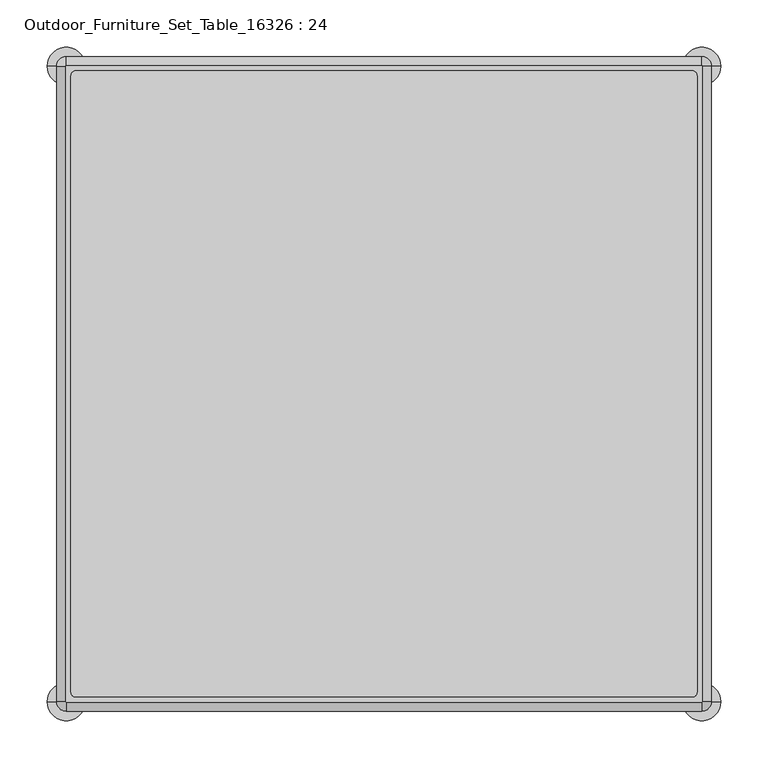
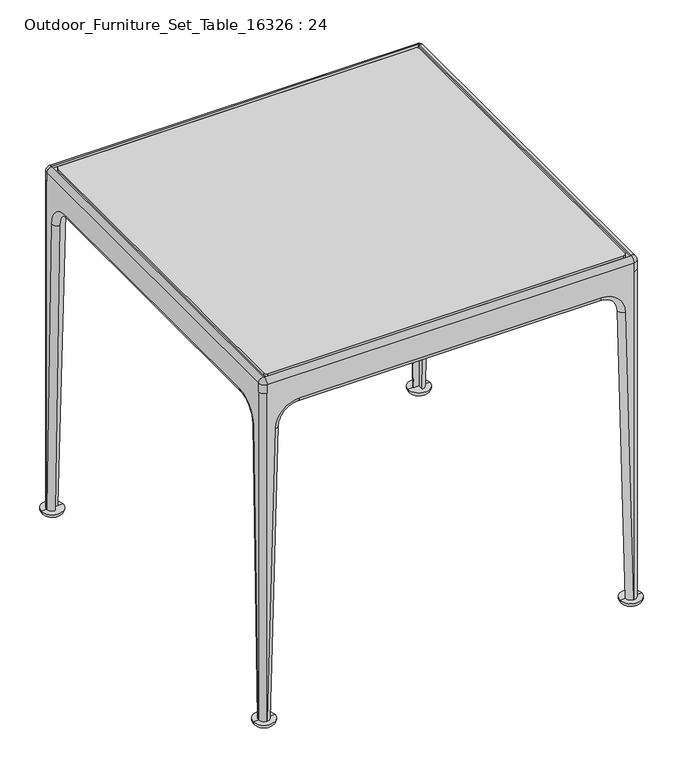
"""IFC4 building model written with IfcOpenShell, lengths in millimetres: furniture geometry, Outdoor_Furniture_Set_Table_16326 : 24."""

from ifc_helpers import new_model, si_unit, point, frame, frame_2d, origin, place, context, project, spatial, polyline, circle_curve, ellipse_curve, trimmed, segment, composite_curve, outline, extrude, source, transform, mapped, element, save
from ifc_brep_helpers import plane_surface, cylinder_surface, revolved_surface, advanced_brep


def outdoor_furniture_set_table_16326_24_87b8b4b7(model_context):
    return source(origin(), model_context, "Body", "SolidModel", [
        extrude(outline(polyline([(337.0, 337.0), (337.0, -337.0), (-337.0, -337.0), (-337.0, 337.0), (337.0, 337.0)])), frame((0.0, 0.0, 645.0), z_axis=(0.0, 0.0, 1.0), x_axis=(1.0, 0.0, 0.0)), (0.0, 0.0, 1.0), 20.0),
        advanced_brep(
        [(-336.0, 346.0, 10.0), (-326.0034268, 336.0, 9.7382305), (-336.0, 336.0, 10.0), (-321.3050379, 346.0, 571.1779627), (-311.3084646, 336.0, 570.9161932), (-276.3204583, 336.0, 605.0), (276.3204583, 336.0, 605.0), (311.3084646, 336.0, 570.9161932), (326.0034268, 336.0, 9.7382305), (336.0, 336.0, 10.0), (336.0, 336.0, 645.0), (-336.0, 336.0, 645.0), (-276.3204583, 346.0, 615.0), (276.3204583, 346.0, 615.0), (321.3050379, 346.0, 571.1779627), (336.0, 346.0, 10.0), (-336.0, 346.0, 645.0), (-336.0, 346.0, 661.0), (336.0, 346.0, 661.0), (336.0, 346.0, 645.0), (-337.0, -336.0, 645.0), (-336.0, -337.0, 645.0), (336.0, -337.0, 645.0), (337.0, -336.0, 645.0), (337.0, 336.0, 645.0), (336.0, 337.0, 645.0), (-336.0, 337.0, 645.0), (-337.0, 336.0, 645.0), (336.0, -336.0, 645.0), (-336.0, -336.0, 645.0), (-336.0, -346.0, 661.0), (-346.0, -336.0, 661.0), (-346.0, -336.0, 645.0), (-336.0, -346.0, 645.0), (-336.0, -337.0, 670.0), (-337.0, -336.0, 670.0), (-336.0, -346.0, 10.0), (-321.3050273, -346.0, 571.1783664), (-276.3204583, -346.0, 615.0), (276.3204583, -346.0, 615.0), (321.3050273, -346.0, 571.1783664), (336.0, -346.0, 10.0), (336.0, -346.0, 645.0), (336.0, -346.0, 661.0), (336.0, -337.0, 670.0), (346.0, -336.0, 645.0), (346.0, -336.0, 661.0), (337.0, -336.0, 670.0), (346.0, -336.0, 10.0), (346.0, -321.3050379, 571.1779627), (346.0, -276.3204583, 615.0), (346.0, 276.3204583, 615.0), (346.0, 321.3050379, 571.1779627), (346.0, 336.0, 10.0), (346.0, 336.0, 645.0), (346.0, 336.0, 661.0), (337.0, 336.0, 670.0), (336.0, 337.0, 670.0), (-336.0, 337.0, 670.0), (-346.0, 336.0, 645.0), (-346.0, 336.0, 661.0), (-337.0, 336.0, 670.0), (-346.0, 336.0, 10.0), (-346.0, 321.3050273, 571.1783665), (-346.0, 276.3208622, 615.0), (-346.0, -276.3208622, 615.0), (-346.0, -321.3050273, 571.1783665), (-346.0, -336.0, 10.0), (-336.0, -326.0034268, 9.7382305), (-336.0, -336.0, 10.0), (-336.0, -311.3084541, 570.916597), (-336.0, -276.3208622, 605.0), (-336.0, 276.3208622, 605.0), (-336.0, 311.3084541, 570.916597), (-336.0, 326.0034268, 9.7382305), (326.0034268, -336.0, 9.7382305), (336.0, -336.0, 10.0), (311.3084564, -336.0, 570.9165072), (276.3204583, -336.0, 605.0), (-276.3204583, -336.0, 605.0), (-311.3084564, -336.0, 570.9165072), (-326.0034268, -336.0, 9.7382305), (336.0, 326.0034268, 9.7382305), (336.0, 311.3084646, 570.9161932), (336.0, 276.3204583, 605.0), (336.0, -276.3204583, 605.0), (336.0, -311.3084646, 570.9161932), (336.0, -326.0034268, 9.7382305)],
        [
            (0, 1, circle_curve(frame((-336.0, 336.0, 10.0), z_axis=(-0.026176948307801547, 0.0, -0.9996573249755591), x_axis=(0.9996573249755591, 0.0, -0.026176948307801547)), 10.0)),
            (1, 2),
            (2, 0),
            (0, 3),
            (3, 4, circle_curve(frame((-321.3050379, 336.0, 571.1779627), z_axis=(-0.026176948307801547, 0.0, -0.9996573249755591), x_axis=(0.9996573249755591, 0.0, -0.026176948307801547)), 10.0)),
            (4, 1),
            (4, 5, circle_curve(frame((-276.3204583, 336.0, 570.0), z_axis=(0.0, 1.0, 0.0), x_axis=(-0.9996573249743329, 0.0, 0.026176948354628502)), 35.0)),
            (5, 6),
            (6, 7, circle_curve(frame((276.3204583, 336.0, 570.0), z_axis=(0.0, 1.0, 0.0), x_axis=(0.0, 0.0, 1.0)), 35.0)),
            (7, 8),
            (8, 9),
            (9, 10),
            (10, 11),
            (11, 2),
            (3, 12, circle_curve(frame((-276.3204583, 346.0, 570.0), z_axis=(0.0, 1.0, 0.0), x_axis=(-0.9996573249743329, 0.0, 0.026176948354628502)), 45.0)),
            (12, 5, circle_curve(frame((-276.3204583, 336.0, 615.0), z_axis=(-1.0, 0.0, 0.0), x_axis=(0.0, 0.0, -1.0)), 10.0)),
            (12, 13),
            (13, 6, circle_curve(frame((276.3204583, 336.0, 615.0), z_axis=(-1.0, 0.0, 0.0), x_axis=(0.0, 0.0, -1.0)), 10.0)),
            (13, 14, circle_curve(frame((276.3204583, 346.0, 570.0), z_axis=(0.0, 1.0, 0.0), x_axis=(0.0, 0.0, 1.0)), 45.0)),
            (14, 7, circle_curve(frame((321.3050379, 336.0, 571.1779627), z_axis=(-0.02617694835452745, 0.0, 0.9996573249743356), x_axis=(-0.9996573249743356, 0.0, -0.02617694835452745)), 10.0)),
            (8, 15, circle_curve(frame((336.0, 336.0, 10.0), z_axis=(0.026176948307803226, 0.0, -0.9996573249755591), x_axis=(-0.9996573249755591, 0.0, -0.026176948307803226)), 10.0)),
            (15, 9),
            (14, 15),
            (0, 16),
            (16, 17),
            (17, 18),
            (18, 19),
            (19, 15),
            (20, 21, circle_curve(frame((-336.0, -336.0, 645.0), z_axis=(0.0, 0.0, 1.0), x_axis=(-1.0, 0.0, 0.0)), 1.0)),
            (21, 22),
            (22, 23, circle_curve(frame((336.0, -336.0, 645.0), z_axis=(0.0, 0.0, 1.0), x_axis=(0.0, -1.0, 0.0)), 1.0)),
            (23, 24),
            (24, 25, circle_curve(frame((336.0, 336.0, 645.0), z_axis=(0.0, 0.0, 1.0), x_axis=(1.0, 0.0, 0.0)), 1.0)),
            (25, 26),
            (26, 27, circle_curve(frame((-336.0, 336.0, 645.0), z_axis=(0.0, 0.0, 1.0), x_axis=(0.0, 1.0, 0.0)), 1.0)),
            (27, 20),
            (10, 28),
            (28, 29),
            (29, 11),
            (30, 31, circle_curve(frame((-336.0, -336.0, 661.0), z_axis=(0.0, 0.0, -1.0), x_axis=(-1.0, 0.0, 0.0)), 10.0)),
            (31, 32),
            (32, 33, circle_curve(frame((-336.0, -336.0, 645.0), z_axis=(0.0, 0.0, 1.0), x_axis=(-1.0, 0.0, 0.0)), 10.0)),
            (33, 30),
            (30, 34, circle_curve(frame((-336.0, -337.0, 661.0), z_axis=(-1.0, 0.0, 0.0), x_axis=(0.0, 1.0, 0.0)), 9.0)),
            (34, 35, circle_curve(frame((-336.0, -336.0, 670.0), z_axis=(0.0, 0.0, -1.0), x_axis=(-1.0, 0.0, 0.0)), 1.0)),
            (35, 31, circle_curve(frame((-337.0, -336.0, 661.0), z_axis=(0.0, -1.0, 0.0), x_axis=(1.0, 0.0, 0.0)), 9.0)),
            (33, 36),
            (36, 37),
            (37, 38, circle_curve(frame((-276.3204583, -346.0, 570.0), z_axis=(0.0, 1.0, 0.0), x_axis=(0.0, 0.0, 1.0)), 45.0)),
            (38, 39),
            (39, 40, circle_curve(frame((276.3204583, -346.0, 570.0), z_axis=(0.0, 1.0, 0.0), x_axis=(0.9996570900025821, 0.0, 0.026185920025262065)), 45.0)),
            (40, 41),
            (41, 42),
            (42, 43),
            (43, 30),
            (43, 44, circle_curve(frame((336.0, -337.0, 661.0), z_axis=(-1.0, 0.0, 0.0), x_axis=(0.0, 1.0, 0.0)), 9.0)),
            (44, 34),
            (42, 45, circle_curve(frame((336.0, -336.0, 645.0), z_axis=(0.0, 0.0, 1.0), x_axis=(0.0, -1.0, 0.0)), 10.0)),
            (45, 46),
            (46, 43, circle_curve(frame((336.0, -336.0, 661.0), z_axis=(0.0, 0.0, -1.0), x_axis=(0.0, -1.0, 0.0)), 10.0)),
            (46, 47, circle_curve(frame((337.0, -336.0, 661.0), z_axis=(0.0, -1.0, 0.0), x_axis=(-1.0, 0.0, 0.0)), 9.0)),
            (47, 44, circle_curve(frame((336.0, -336.0, 670.0), z_axis=(0.0, 0.0, -1.0), x_axis=(0.0, -1.0, 0.0)), 1.0)),
            (45, 48),
            (48, 49),
            (49, 50, circle_curve(frame((346.0, -276.3204583, 570.0), z_axis=(-1.0, 0.0, 0.0), x_axis=(0.0, 0.0, 1.0)), 45.0)),
            (50, 51),
            (51, 52, circle_curve(frame((346.0, 276.3204583, 570.0), z_axis=(-1.0, 0.0, 0.0), x_axis=(0.0, 0.9996573249744088, 0.026176948351728707)), 45.0)),
            (52, 53),
            (53, 54),
            (54, 55),
            (55, 46),
            (55, 56, circle_curve(frame((337.0, 336.0, 661.0), z_axis=(0.0, -1.0, 0.0), x_axis=(-1.0, 0.0, 0.0)), 9.0)),
            (56, 47),
            (54, 19, circle_curve(frame((336.0, 336.0, 645.0), z_axis=(0.0, 0.0, 1.0), x_axis=(1.0, 0.0, 0.0)), 10.0)),
            (18, 55, circle_curve(frame((336.0, 336.0, 661.0), z_axis=(0.0, 0.0, -1.0), x_axis=(1.0, 0.0, 0.0)), 10.0)),
            (18, 57, circle_curve(frame((336.0, 337.0, 661.0), z_axis=(1.0, 0.0, 0.0), x_axis=(0.0, -1.0, 0.0)), 9.0)),
            (57, 56, circle_curve(frame((336.0, 336.0, 670.0), z_axis=(0.0, 0.0, -1.0), x_axis=(1.0, 0.0, 0.0)), 1.0)),
            (17, 58, circle_curve(frame((-336.0, 337.0, 661.0), z_axis=(1.0, 0.0, 0.0), x_axis=(0.0, -1.0, 0.0)), 9.0)),
            (58, 57),
            (16, 59, circle_curve(frame((-336.0, 336.0, 645.0), z_axis=(0.0, 0.0, 1.0), x_axis=(0.0, 1.0, 0.0)), 10.0)),
            (59, 60),
            (60, 17, circle_curve(frame((-336.0, 336.0, 661.0), z_axis=(0.0, 0.0, -1.0), x_axis=(0.0, 1.0, 0.0)), 10.0)),
            (60, 61, circle_curve(frame((-337.0, 336.0, 661.0), z_axis=(0.0, 1.0, 0.0), x_axis=(1.0, 0.0, 0.0)), 9.0)),
            (61, 58, circle_curve(frame((-336.0, 336.0, 670.0), z_axis=(0.0, 0.0, -1.0), x_axis=(0.0, 1.0, 0.0)), 1.0)),
            (31, 60),
            (59, 62),
            (62, 63),
            (63, 64, circle_curve(frame((-346.0, 276.3208622, 570.0004146), z_axis=(1.0, 0.0, 0.0), x_axis=(0.0, 0.0, 1.0)), 44.9995854)),
            (64, 65),
            (65, 66, circle_curve(frame((-346.0, -276.3208622, 570.0004146), z_axis=(1.0, 0.0, 0.0), x_axis=(0.0, -0.9996573249744442, 0.026176948350383943)), 44.9995854)),
            (66, 67),
            (67, 32),
            (35, 61),
            (34, 21),
            (20, 35),
            (44, 22),
            (47, 23),
            (56, 24),
            (57, 25),
            (58, 26),
            (61, 27),
            (67, 68, circle_curve(frame((-336.0, -336.0, 10.0), z_axis=(0.0, -0.0261769483078763, -0.9996573249755573), x_axis=(0.0, -0.9996573249755573, 0.0261769483078763)), 10.0)),
            (68, 69),
            (69, 67),
            (66, 70, circle_curve(frame((-336.0, -321.3050273, 571.1783665), z_axis=(0.0, -0.0261769483078763, -0.9996573249755573), x_axis=(0.0, -0.9996573249755573, 0.0261769483078763)), 10.0)),
            (70, 68),
            (70, 71, circle_curve(frame((-336.0, -276.3208622, 570.0004146), z_axis=(-1.0, 0.0, 0.0), x_axis=(0.0, -0.9996573249744442, 0.026176948350383943)), 34.9995854)),
            (71, 72),
            (72, 73, circle_curve(frame((-336.0, 276.3208622, 570.0004146), z_axis=(-1.0, 0.0, 0.0), x_axis=(0.0, 0.0, 1.0)), 34.9995854)),
            (73, 74),
            (74, 2),
            (29, 69),
            (65, 71, circle_curve(frame((-336.0, -276.3208622, 615.0), z_axis=(0.0, -1.0, 0.0), x_axis=(0.0, 0.0, 1.0)), 10.0)),
            (64, 72, circle_curve(frame((-336.0, 276.3208622, 615.0), z_axis=(0.0, -1.0, 0.0), x_axis=(0.0, 0.0, 1.0)), 10.0)),
            (63, 73, circle_curve(frame((-336.0, 321.3050273, 571.1783665), z_axis=(0.0, -0.026176948350192727, 0.9996573249744491), x_axis=(0.0, 0.9996573249744491, 0.026176948350192727)), 10.0)),
            (74, 62, circle_curve(frame((-336.0, 336.0, 10.0), z_axis=(0.0, 0.026176948307874842, -0.9996573249755573), x_axis=(0.0, 0.9996573249755573, 0.026176948307874842)), 10.0)),
            (62, 2),
            (41, 75, circle_curve(frame((336.0, -336.0, 10.0), z_axis=(0.02617694831120199, 0.0, -0.9996573249754701), x_axis=(-0.9996573249754701, 0.0, -0.02617694831120199)), 10.0)),
            (75, 76),
            (76, 41),
            (40, 77, circle_curve(frame((321.3050273, -336.0, 571.1783664), z_axis=(0.026185920025262068, 0.0, -0.9996570900025821), x_axis=(-0.9996570900025821, 0.0, -0.026185920025262068)), 10.0)),
            (77, 75),
            (77, 78, circle_curve(frame((276.3204583, -336.0, 570.0), z_axis=(0.0, -1.0, 0.0), x_axis=(0.9996570900025821, 0.0, 0.026185920025262065)), 35.0)),
            (78, 79),
            (79, 80, circle_curve(frame((-276.3204583, -336.0, 570.0), z_axis=(0.0, -1.0, 0.0), x_axis=(0.0, 0.0, 1.0)), 35.0)),
            (80, 81),
            (81, 69),
            (28, 76),
            (39, 78, circle_curve(frame((276.3204583, -336.0, 615.0), z_axis=(1.0, 0.0, 0.0), x_axis=(0.0, 0.0, -1.0)), 10.0)),
            (38, 79, circle_curve(frame((-276.3204583, -336.0, 615.0), z_axis=(1.0, 0.0, 0.0), x_axis=(0.0, 0.0, -1.0)), 10.0)),
            (37, 80, circle_curve(frame((-321.3050273, -336.0, 571.1783664), z_axis=(0.02618592008575971, 0.0, 0.9996570900009975), x_axis=(0.9996570900009975, 0.0, -0.02618592008575971)), 10.0)),
            (81, 36, circle_curve(frame((-336.0, -336.0, 10.0), z_axis=(-0.026176948310976122, 0.0, -0.999657324975476), x_axis=(0.999657324975476, 0.0, -0.026176948310976122)), 10.0)),
            (36, 69),
            (53, 82, circle_curve(frame((336.0, 336.0, 10.0), z_axis=(0.0, 0.026176948307689504, -0.9996573249755621), x_axis=(0.0, -0.9996573249755621, -0.026176948307689504)), 10.0)),
            (82, 9),
            (9, 53),
            (52, 83, circle_curve(frame((336.0, 321.3050379, 571.1779627), z_axis=(0.0, 0.026176948307689504, -0.9996573249755621), x_axis=(0.0, -0.9996573249755621, -0.026176948307689504)), 10.0)),
            (83, 82),
            (83, 84, circle_curve(frame((336.0, 276.3204583, 570.0), z_axis=(1.0, 0.0, 0.0), x_axis=(0.0, 0.9996573249744088, 0.026176948351728707)), 35.0)),
            (84, 85),
            (85, 86, circle_curve(frame((336.0, -276.3204583, 570.0), z_axis=(1.0, 0.0, 0.0), x_axis=(0.0, 0.0, 1.0)), 35.0)),
            (86, 87),
            (87, 76),
            (51, 84, circle_curve(frame((336.0, 276.3204583, 615.0), z_axis=(0.0, 0.9999999999999999, 0.0), x_axis=(0.0, 0.0, -0.9999999999999999)), 10.0)),
            (50, 85, circle_curve(frame((336.0, -276.3204583, 615.0), z_axis=(0.0, 1.0, 0.0), x_axis=(0.0, 0.0, -1.0)), 10.0)),
            (49, 86, circle_curve(frame((336.0, -321.3050379, 571.1779627), z_axis=(0.0, 0.026176948354554516, 0.9996573249743349), x_axis=(0.0, 0.9996573249743349, -0.026176948354554516)), 10.0)),
            (87, 48, circle_curve(frame((336.0, -336.0, 10.0), z_axis=(0.0, -0.02617694830776857, -0.99965732497556), x_axis=(0.0, 0.99965732497556, -0.02617694830776857)), 10.0)),
            (48, 76),
            (15, 53, circle_curve(frame((336.0, 336.0, 10.0), z_axis=(0.0, 0.0, -1.0), x_axis=(1.0, 0.0, 0.0)), 10.0)),
            (48, 41, circle_curve(frame((336.0, -336.0, 10.0), z_axis=(0.0, 0.0, -1.0), x_axis=(1.0, 0.0, 0.0)), 10.0)),
            (36, 67, circle_curve(frame((-336.0, -336.0, 10.0), z_axis=(0.0, 0.0, -1.0), x_axis=(1.0, 0.0, 0.0)), 10.0)),
            (62, 0, circle_curve(frame((-336.0, 336.0, 10.0), z_axis=(0.0, 0.0, -1.0), x_axis=(1.0, 0.0, 0.0)), 10.0)),
        ],
        [
            plane_surface(frame((-336.0, 346.0, 10.0), z_axis=(-0.026176948307801547, 0.0, -0.9996573249755591), x_axis=(0.0, 1.0, 0.0))),
            cylinder_surface(frame((-336.0, 336.0, 10.0), z_axis=(-0.026176948307801547, 0.0, -0.9996573249755591), x_axis=(0.9996573249755591, 0.0, -0.026176948307801547)), 10.0),
            plane_surface(frame((-326.0034268, 336.0, 9.7382305), z_axis=(0.0, -1.0, 0.0), x_axis=(0.026176948307801564, 0.0, 0.9996573249755591))),
            revolved_surface(trimmed(ellipse_curve(frame((-321.3050379, 336.0, 571.1779627), z_axis=(-0.026176948354628502, 0.0, -0.9996573249743329), x_axis=(0.9996573249743329, 0.0, -0.026176948354628502)), 10.0, 10.0), [point((-321.3050379, 346.0, 571.1779627))], [point((-311.3084646, 336.0, 570.9161932))], True, "CARTESIAN"), (-276.3204583, 346.0, 570.0), (0.0, 1.0, 0.0)),
            cylinder_surface(frame((-276.3204583, 336.0, 615.0), z_axis=(-1.0, 0.0, 0.0), x_axis=(0.0, 0.0, -1.0)), 10.0),
            revolved_surface(trimmed(ellipse_curve(frame((276.3204583, 336.0, 615.0), z_axis=(-1.0, 0.0, 0.0), x_axis=(0.0, 0.0, -1.0)), 10.0, 10.0), [point((276.3204583, 346.0, 615.0))], [point((276.3204583, 336.0, 605.0))], True, "CARTESIAN"), (276.3204583, 346.0, 570.0), (0.0, 1.0, 0.0)),
            plane_surface(frame((336.0, 346.0, 10.0), z_axis=(0.026176948307803226, 0.0, -0.9996573249755591), x_axis=(0.0, 1.0, 0.0))),
            cylinder_surface(frame((321.3050379, 336.0, 571.1779627), z_axis=(-0.026176948307803226, 0.0, 0.9996573249755591), x_axis=(-0.9996573249755591, 0.0, -0.026176948307803226)), 10.0),
            plane_surface(frame((-276.3204583, 346.0, 615.0), z_axis=(0.0, 1.0, 0.0), x_axis=(-1.0, 0.0, 0.0))),
            plane_surface(frame((-336.0, 346.0, 645.0), z_axis=(0.0, 0.0, 1.0), x_axis=(0.0, -1.0, 0.0))),
            cylinder_surface(frame((-336.0, -336.0, 0.0), z_axis=(0.0, 0.0, 1.0), x_axis=(-1.0, 0.0, 0.0)), 10.0),
            revolved_surface(trimmed(ellipse_curve(frame((-337.0, -336.0, 661.0), z_axis=(0.0, 1.0, 0.0), x_axis=(1.0, 0.0, 0.0)), 9.0, 9.0), [point((-346.0, -336.0, 661.0))], [point((-337.0, -336.0, 670.0))], True, "CARTESIAN"), (-336.0, -336.0, 0.0), (0.0, 0.0, 1.0)),
            plane_surface(frame((-336.0, -346.0, 645.0), z_axis=(0.0, -1.0, 0.0), x_axis=(1.0, 0.0, 0.0))),
            cylinder_surface(frame((-336.0, -337.0, 661.0), z_axis=(-1.0, 0.0, 0.0), x_axis=(0.0, 1.0, 0.0)), 9.0),
            cylinder_surface(frame((336.0, -336.0, 0.0), z_axis=(0.0, 0.0, 1.0), x_axis=(0.0, -1.0, 0.0)), 10.0),
            revolved_surface(trimmed(ellipse_curve(frame((336.0, -337.0, 661.0), z_axis=(-1.0, 0.0, 0.0), x_axis=(0.0, 1.0, 0.0)), 9.0, 9.0), [point((336.0, -346.0, 661.0))], [point((336.0, -337.0, 670.0))], True, "CARTESIAN"), (336.0, -336.0, 0.0), (0.0, 0.0, 1.0)),
            plane_surface(frame((346.0, -336.0, 645.0), z_axis=(1.0, 0.0, 0.0), x_axis=(0.0, 1.0, 0.0))),
            cylinder_surface(frame((337.0, -336.0, 661.0), z_axis=(0.0, -1.0, 0.0), x_axis=(-1.0, 0.0, 0.0)), 9.0),
            cylinder_surface(frame((336.0, 336.0, 0.0), z_axis=(0.0, 0.0, 1.0), x_axis=(1.0, 0.0, 0.0)), 10.0),
            revolved_surface(trimmed(ellipse_curve(frame((337.0, 336.0, 661.0), z_axis=(0.0, -1.0, 0.0), x_axis=(-1.0, 0.0, 0.0)), 9.0, 9.0), [point((346.0, 336.0, 661.0))], [point((337.0, 336.0, 670.0))], True, "CARTESIAN"), (336.0, 336.0, 0.0), (0.0, 0.0, 1.0)),
            cylinder_surface(frame((336.0, 337.0, 661.0), z_axis=(1.0, 0.0, 0.0), x_axis=(0.0, -1.0, 0.0)), 9.0),
            cylinder_surface(frame((-336.0, 336.0, 0.0), z_axis=(0.0, 0.0, 1.0), x_axis=(0.0, 1.0, 0.0)), 10.0),
            revolved_surface(trimmed(ellipse_curve(frame((-336.0, 337.0, 661.0), z_axis=(1.0, 0.0, 0.0), x_axis=(0.0, -1.0, 0.0)), 9.0, 9.0), [point((-336.0, 346.0, 661.0))], [point((-336.0, 337.0, 670.0))], True, "CARTESIAN"), (-336.0, 336.0, 0.0), (0.0, 0.0, 1.0)),
            plane_surface(frame((-346.0, 336.0, 645.0), z_axis=(-1.0, 0.0, 0.0), x_axis=(0.0, -1.0, 0.0))),
            cylinder_surface(frame((-337.0, 336.0, 661.0), z_axis=(0.0, 1.0, 0.0), x_axis=(1.0, 0.0, 0.0)), 9.0),
            revolved_surface(polyline([(-337.0, -336.0, 670.0), (-337.0, -336.0, 645.0)]), (-336.0, -336.0, 0.0), (0.0, 0.0, 1.0)),
            plane_surface(frame((-336.0, -337.0, 670.0), z_axis=(0.0, 1.0, 0.0), x_axis=(1.0, 0.0, 0.0))),
            revolved_surface(polyline([(336.0, -337.0, 670.0), (336.0, -337.0, 645.0)]), (336.0, -336.0, 0.0), (0.0, 0.0, 1.0)),
            plane_surface(frame((337.0, -336.0, 670.0), z_axis=(-1.0, 0.0, 0.0), x_axis=(0.0, 1.0, 0.0))),
            revolved_surface(polyline([(337.0, 336.0, 670.0), (337.0, 336.0, 645.0)]), (336.0, 336.0, 0.0), (0.0, 0.0, 1.0)),
            plane_surface(frame((336.0, 337.0, 670.0), z_axis=(0.0, -1.0, 0.0), x_axis=(-1.0, 0.0, 0.0))),
            revolved_surface(polyline([(-336.0, 337.0, 670.0), (-336.0, 337.0, 645.0)]), (-336.0, 336.0, 0.0), (0.0, 0.0, 1.0)),
            plane_surface(frame((-337.0, 336.0, 670.0), z_axis=(1.0, 0.0, 0.0), x_axis=(0.0, -1.0, 0.0))),
            plane_surface(frame((-346.0, -336.0, 10.0), z_axis=(0.0, -0.0261769483078763, -0.9996573249755573), x_axis=(1.0, 0.0, 0.0))),
            cylinder_surface(frame((-336.0, -336.0, 10.0), z_axis=(0.0, -0.0261769483078763, -0.9996573249755573), x_axis=(0.0, -0.9996573249755573, 0.0261769483078763)), 10.0),
            plane_surface(frame((-336.0, -326.0034268, 9.7382305), z_axis=(1.0, 0.0, 0.0), x_axis=(0.0, 0.026176948307876334, 0.9996573249755573))),
            revolved_surface(trimmed(ellipse_curve(frame((-336.0, -321.3050273, 571.1783665), z_axis=(0.0, -0.026176948350383943, -0.9996573249744442), x_axis=(0.0, -0.9996573249744442, 0.026176948350383943)), 10.0, 10.0), [point((-346.0, -321.3050273, 571.1783665))], [point((-336.0, -311.3084541, 570.916597))], True, "CARTESIAN"), (-346.0, -276.3208622, 570.0004146), (-1.0, 0.0, 0.0)),
            cylinder_surface(frame((-336.0, -276.3208622, 615.0), z_axis=(0.0, -1.0, 0.0), x_axis=(0.0, 0.0, 1.0)), 10.0),
            revolved_surface(trimmed(ellipse_curve(frame((-336.0, 276.3208622, 615.0), z_axis=(0.0, -1.0, 0.0), x_axis=(0.0, 0.0, 1.0)), 10.0, 10.0), [point((-346.0, 276.3208622, 615.0))], [point((-336.0, 276.3208622, 605.0))], True, "CARTESIAN"), (-346.0, 276.3208622, 570.0004146), (-1.0, 0.0, 0.0)),
            plane_surface(frame((-346.0, 336.0, 10.0), z_axis=(0.0, 0.026176948307874842, -0.9996573249755573), x_axis=(1.0, 0.0, 0.0))),
            cylinder_surface(frame((-336.0, 321.3050273, 571.1783665), z_axis=(0.0, -0.026176948307874842, 0.9996573249755573), x_axis=(0.0, 0.9996573249755573, 0.026176948307874842)), 10.0),
            plane_surface(frame((336.0, -346.0, 10.0), z_axis=(0.02617694831120199, 0.0, -0.9996573249754701), x_axis=(0.0, -1.0, 0.0))),
            cylinder_surface(frame((336.0, -336.0, 10.0), z_axis=(0.02617694831120199, 0.0, -0.9996573249754701), x_axis=(-0.9996573249754701, 0.0, -0.02617694831120199)), 10.0),
            plane_surface(frame((326.0034268, -336.0, 9.7382305), z_axis=(0.0, 1.0, 0.0), x_axis=(-0.026176948311202, 0.0, 0.9996573249754701))),
            revolved_surface(trimmed(ellipse_curve(frame((321.3050273, -336.0, 571.1783664), z_axis=(0.026185920025262068, 0.0, -0.9996570900025821), x_axis=(-0.9996570900025821, 0.0, -0.026185920025262068)), 10.0, 10.0), [point((321.3050273, -346.0, 571.1783664))], [point((311.3084564, -336.0, 570.9165072))], True, "CARTESIAN"), (276.3204583, -346.0, 570.0), (0.0, -1.0, 0.0)),
            cylinder_surface(frame((276.3204583, -336.0, 615.0), z_axis=(1.0, 0.0, 0.0), x_axis=(0.0, 0.0, -1.0)), 10.0),
            revolved_surface(trimmed(ellipse_curve(frame((-276.3204583, -336.0, 615.0), z_axis=(1.0, 0.0, 0.0), x_axis=(0.0, 0.0, -1.0)), 10.0, 10.0), [point((-276.3204583, -346.0, 615.0))], [point((-276.3204583, -336.0, 605.0))], True, "CARTESIAN"), (-276.3204583, -346.0, 570.0), (0.0, -1.0, 0.0)),
            plane_surface(frame((-336.0, -346.0, 10.0), z_axis=(-0.026176948310976125, 0.0, -0.999657324975476), x_axis=(0.0, -1.0, 0.0))),
            cylinder_surface(frame((-321.3050273, -336.0, 571.1783664), z_axis=(0.026176948310976122, 0.0, 0.999657324975476), x_axis=(0.999657324975476, 0.0, -0.026176948310976122)), 10.0),
            plane_surface(frame((346.0, 336.0, 10.0), z_axis=(0.0, 0.026176948307689504, -0.9996573249755621), x_axis=(1.0, 0.0, 0.0))),
            cylinder_surface(frame((336.0, 336.0, 10.0), z_axis=(0.0, 0.026176948307689504, -0.9996573249755621), x_axis=(0.0, -0.9996573249755621, -0.026176948307689504)), 10.0),
            plane_surface(frame((336.0, 326.0034268, 9.7382305), z_axis=(-1.0, 0.0, 0.0), x_axis=(0.0, -0.02617694830768952, 0.9996573249755621))),
            revolved_surface(trimmed(ellipse_curve(frame((336.0, 321.3050379, 571.1779627), z_axis=(0.0, 0.0261769483517287, -0.9996573249744088), x_axis=(0.0, -0.9996573249744088, -0.0261769483517287)), 10.0, 10.0), [point((346.0, 321.3050379, 571.1779627))], [point((336.0, 311.3084646, 570.9161932))], True, "CARTESIAN"), (346.0, 276.3204583, 570.0), (1.0, 0.0, 0.0)),
            cylinder_surface(frame((336.0, 276.3204583, 615.0), z_axis=(0.0, 1.0, 0.0), x_axis=(0.0, 0.0, -1.0)), 10.0),
            revolved_surface(trimmed(ellipse_curve(frame((336.0, -276.3204583, 615.0), z_axis=(0.0, 1.0, 0.0), x_axis=(0.0, 0.0, -1.0)), 10.0, 10.0), [point((346.0, -276.3204583, 615.0))], [point((336.0, -276.3204583, 605.0))], True, "CARTESIAN"), (346.0, -276.3204583, 570.0), (1.0, 0.0, 0.0)),
            plane_surface(frame((346.0, -336.0, 10.0), z_axis=(0.0, -0.026176948307768563, -0.99965732497556), x_axis=(1.0, 0.0, 0.0))),
            cylinder_surface(frame((336.0, -321.3050379, 571.1779627), z_axis=(0.0, 0.02617694830776857, 0.99965732497556), x_axis=(0.0, 0.99965732497556, -0.02617694830776857)), 10.0),
            plane_surface(frame((336.0, 336.0, 10.0), z_axis=(0.0, 0.0, -1.0), x_axis=(-1.0, 0.0, 0.0))),
            cylinder_surface(frame((336.0, 336.0, 10.0), z_axis=(0.0, 0.0, 1.0), x_axis=(1.0, 0.0, 0.0)), 10.0),
            cylinder_surface(frame((336.0, -336.0, 0.0), z_axis=(0.0, 0.0, 1.0), x_axis=(1.0, 0.0, 0.0)), 10.0),
            cylinder_surface(frame((-336.0, -336.0, 0.0), z_axis=(0.0, 0.0, 1.0), x_axis=(1.0, 0.0, 0.0)), 10.0),
            cylinder_surface(frame((-336.0, 336.0, 0.0), z_axis=(0.0, 0.0, 1.0), x_axis=(1.0, 0.0, 0.0)), 10.0),
        ],
        [
            (0, [[1, 2, 3]]),
            (1, [[-1, 4, 5, 6]]),
            (2, [[-2, -6, 7, 8, 9, 10, 11, 12, 13, 14]]),
            (3, [[-5, 15, 16, -7]]),
            (4, [[-8, -16, 17, 18]]),
            (5, [[-9, -18, 19, 20]]),
            (6, [[-11, 21, 22]]),
            (7, [[-10, -20, 23, -21]]),
            (8, [[-4, 24, 25, 26, 27, 28, -23, -19, -17, -15]]),
            (9, [[29, 30, 31, 32, 33, 34, 35, 36], [-13, 37, 38, 39]]),
            (10, [[40, 41, 42, 43]]),
            (11, [[-40, 44, 45, 46]]),
            (12, [[-43, 47, 48, 49, 50, 51, 52, 53, 54, 55]]),
            (13, [[-44, -55, 56, 57]]),
            (14, [[-54, 58, 59, 60]]),
            (15, [[-56, -60, 61, 62]]),
            (16, [[-59, 63, 64, 65, 66, 67, 68, 69, 70, 71]]),
            (17, [[-61, -71, 72, 73]]),
            (18, [[-70, 74, -27, 75]]),
            (19, [[-72, -75, 76, 77]]),
            (20, [[-76, -26, 78, 79]]),
            (21, [[-25, 80, 81, 82]]),
            (22, [[-78, -82, 83, 84]]),
            (23, [[-41, 85, -81, 86, 87, 88, 89, 90, 91, 92]]),
            (24, [[-46, 93, -83, -85]]),
            (25, [[-45, 94, -29, 95]]),
            (26, [[-57, 96, -30, -94]]),
            (27, [[-62, 97, -31, -96]]),
            (28, [[-73, 98, -32, -97]]),
            (29, [[-77, 99, -33, -98]]),
            (30, [[-79, 100, -34, -99]]),
            (31, [[-84, 101, -35, -100]]),
            (32, [[-93, -95, -36, -101]]),
            (33, [[102, 103, 104]]),
            (34, [[-102, -91, 105, 106]]),
            (35, [[-103, -106, 107, 108, 109, 110, 111, -14, -39, 112]]),
            (36, [[-105, -90, 113, -107]]),
            (37, [[-108, -113, -89, 114]]),
            (38, [[-109, -114, -88, 115]]),
            (39, [[-111, 116, 117]]),
            (40, [[-110, -115, -87, -116]]),
            (41, [[118, 119, 120]]),
            (42, [[-118, -52, 121, 122]]),
            (43, [[-119, -122, 123, 124, 125, 126, 127, -112, -38, 128]]),
            (44, [[-121, -51, 129, -123]]),
            (45, [[-124, -129, -50, 130]]),
            (46, [[-125, -130, -49, 131]]),
            (47, [[-127, 132, 133]]),
            (48, [[-126, -131, -48, -132]]),
            (49, [[134, 135, 136]]),
            (50, [[-134, -68, 137, 138]]),
            (51, [[-135, -138, 139, 140, 141, 142, 143, -128, -37, -12]]),
            (52, [[-137, -67, 144, -139]]),
            (53, [[-140, -144, -66, 145]]),
            (54, [[-141, -145, -65, 146]]),
            (55, [[-143, 147, 148]]),
            (56, [[-142, -146, -64, -147]]),
            (57, [[149, -136, -22]]),
            (57, [[150, -120, -148]]),
            (57, [[151, -104, -133]]),
            (57, [[152, -3, -117]]),
            (58, [[-149, -28, -74, -69]]),
            (59, [[-150, -63, -58, -53]]),
            (60, [[-151, -47, -42, -92]]),
            (61, [[-152, -86, -80, -24]]),
        ],
    ),
        extrude(outline(composite_curve([segment(polyline([(326.0228318, -331.0), (-326.0, -331.0)]), True, "CONTINUOUS"), segment(trimmed(circle_curve(frame_2d((-326.0, -326.0)), 5.0), [point((-326.0, -331.0))], [point((-331.0, -326.0))], False, "CARTESIAN"), True, "CONTINUOUS"), segment(polyline([(-331.0, -326.0), (-331.0, 326.0)]), True, "CONTINUOUS"), segment(trimmed(circle_curve(frame_2d((-326.0, 326.0)), 5.0), [point((-331.0, 326.0))], [point((-326.0, 331.0))], False, "CARTESIAN"), True, "CONTINUOUS"), segment(polyline([(-326.0, 331.0), (326.0228318, 331.0)]), True, "CONTINUOUS"), segment(trimmed(circle_curve(frame_2d((326.0228318, 326.0)), 5.0), [point((326.0228318, 331.0))], [point((331.0228318, 326.0))], False, "CARTESIAN"), True, "CONTINUOUS"), segment(polyline([(331.0228318, 326.0), (331.0228318, -326.0)]), True, "CONTINUOUS"), segment(trimmed(circle_curve(frame_2d((326.0228318, -326.0)), 5.0), [point((331.0228318, -326.0))], [point((326.0228318, -331.0))], False, "CARTESIAN"), True, "CONTINUOUS")], self_intersect=False)), frame((0.0, 0.0, 665.0), z_axis=(0.0, 0.0, 1.0), x_axis=(1.0, 0.0, 0.0)), (0.0, 0.0, 1.0), 5.0),
        advanced_brep(
        [(-316.0, -336.0, 10.0), (-356.0, -336.0, 10.0), (-336.0, -336.0, 10.0), (-326.0, -336.0, 0.0), (-346.0, -336.0, 0.0), (-336.0, -336.0, 0.0)],
        [
            (0, 1, circle_curve(frame((-336.0, -336.0, 10.0), z_axis=(0.0, 0.0, 1.0), x_axis=(-1.0, 0.0, 0.0)), 20.0)),
            (1, 2),
            (2, 0),
            (1, 0, circle_curve(frame((-336.0, -336.0, 10.0), z_axis=(0.0, 0.0, 1.0), x_axis=(-1.0, 0.0, 0.0)), 20.0)),
            (3, 4, circle_curve(frame((-336.0, -336.0, 0.0), z_axis=(0.0, 0.0, 1.0), x_axis=(-1.0, 0.0, 0.0)), 10.0)),
            (4, 1, circle_curve(frame((-346.0, -336.0, 10.0), z_axis=(0.0, 1.0, 0.0), x_axis=(-1.0, 0.0, 0.0)), 10.0)),
            (0, 3, circle_curve(frame((-326.0, -336.0, 10.0), z_axis=(0.0, 1.0, 0.0), x_axis=(1.0, 0.0, 0.0)), 10.0)),
            (4, 3, circle_curve(frame((-336.0, -336.0, 0.0), z_axis=(0.0, 0.0, 1.0), x_axis=(-1.0, 0.0, 0.0)), 10.0)),
            (5, 4),
            (3, 5),
        ],
        [
            plane_surface(frame((-336.0, -336.0, 10.0), z_axis=(0.0, 0.0, 1.0), x_axis=(-1.0, 0.0, 0.0))),
            revolved_surface(trimmed(ellipse_curve(frame((-346.0, -336.0, 10.0), z_axis=(0.0, -1.0, 0.0), x_axis=(-1.0, 0.0, 0.0)), 10.0, 10.0), [point((-356.0, -336.0, 10.0))], [point((-346.0, -336.0, 0.0))], True, "CARTESIAN"), (-336.0, -336.0, 2718.4), (0.0, 0.0, -1.0)),
            plane_surface(frame((-336.0, -336.0, 0.0), z_axis=(0.0, 0.0, -1.0), x_axis=(-1.0, 0.0, 0.0))),
        ],
        [
            (0, [[1, 2, 3]]),
            (0, [[4, -3, -2]]),
            (1, [[5, 6, -1, 7]]),
            (1, [[8, -7, -4, -6]]),
            (2, [[9, -5, 10]]),
            (2, [[-10, -8, -9]]),
        ],
    ),
        advanced_brep(
        [(326.0, -336.0, 0.0), (346.0, -336.0, 0.0), (336.0, -336.0, 0.0), (316.0, -336.0, 10.0), (356.0, -336.0, 10.0), (336.0, -336.0, 10.0)],
        [
            (0, 1, circle_curve(frame((336.0, -336.0, 0.0), z_axis=(0.0, 0.0, -1.0), x_axis=(1.0, 0.0, 0.0)), 10.0)),
            (1, 2),
            (2, 0),
            (1, 0, circle_curve(frame((336.0, -336.0, 0.0), z_axis=(0.0, 0.0, -1.0), x_axis=(1.0, 0.0, 0.0)), 10.0)),
            (3, 4, circle_curve(frame((336.0, -336.0, 10.0), z_axis=(0.0, 0.0, -1.0), x_axis=(1.0, 0.0, 0.0)), 20.0)),
            (4, 1, circle_curve(frame((346.0, -336.0, 10.0), z_axis=(0.0, 1.0, 0.0), x_axis=(-1.0, 0.0, 0.0)), 10.0)),
            (0, 3, circle_curve(frame((326.0, -336.0, 10.0), z_axis=(0.0, 1.0, 0.0), x_axis=(1.0, 0.0, 0.0)), 10.0)),
            (4, 3, circle_curve(frame((336.0, -336.0, 10.0), z_axis=(0.0, 0.0, -1.0), x_axis=(1.0, 0.0, 0.0)), 20.0)),
            (5, 4),
            (3, 5),
        ],
        [
            plane_surface(frame((336.0, -336.0, 0.0), z_axis=(0.0, 0.0, -1.0), x_axis=(1.0, 0.0, 0.0))),
            revolved_surface(trimmed(ellipse_curve(frame((346.0, -336.0, 10.0), z_axis=(0.0, -1.0, 0.0), x_axis=(-1.0, 0.0, 0.0)), 10.0, 10.0), [point((346.0, -336.0, 0.0))], [point((356.0, -336.0, 10.0))], True, "CARTESIAN"), (336.0, -336.0, 2718.4), (0.0, 0.0, 1.0)),
            plane_surface(frame((336.0, -336.0, 10.0), z_axis=(0.0, 0.0, 1.0), x_axis=(1.0, 0.0, 0.0))),
        ],
        [
            (0, [[1, 2, 3]]),
            (0, [[4, -3, -2]]),
            (1, [[5, 6, -1, 7]]),
            (1, [[8, -7, -4, -6]]),
            (2, [[9, -5, 10]]),
            (2, [[-10, -8, -9]]),
        ],
    ),
        advanced_brep(
        [(316.0, 336.0, 10.0), (356.0, 336.0, 10.0), (336.0, 336.0, 10.0), (326.0, 336.0, 0.0), (346.0, 336.0, 0.0), (336.0, 336.0, 0.0)],
        [
            (0, 1, circle_curve(frame((336.0, 336.0, 10.0), z_axis=(0.0, 0.0, 1.0), x_axis=(1.0, 0.0, 0.0)), 20.0)),
            (1, 2),
            (2, 0),
            (1, 0, circle_curve(frame((336.0, 336.0, 10.0), z_axis=(0.0, 0.0, 1.0), x_axis=(1.0, 0.0, 0.0)), 20.0)),
            (3, 4, circle_curve(frame((336.0, 336.0, 0.0), z_axis=(0.0, 0.0, 1.0), x_axis=(1.0, 0.0, 0.0)), 10.0)),
            (4, 1, circle_curve(frame((346.0, 336.0, 10.0), z_axis=(0.0, -1.0, 0.0), x_axis=(-1.0, 0.0, 0.0)), 10.0)),
            (0, 3, circle_curve(frame((326.0, 336.0, 10.0), z_axis=(0.0, -1.0, 0.0), x_axis=(1.0, 0.0, 0.0)), 10.0)),
            (4, 3, circle_curve(frame((336.0, 336.0, 0.0), z_axis=(0.0, 0.0, 1.0), x_axis=(1.0, 0.0, 0.0)), 10.0)),
            (5, 4),
            (3, 5),
        ],
        [
            plane_surface(frame((336.0, 336.0, 10.0), z_axis=(0.0, 0.0, 1.0), x_axis=(1.0, 0.0, 0.0))),
            revolved_surface(trimmed(ellipse_curve(frame((346.0, 336.0, 10.0), z_axis=(0.0, 1.0, 0.0), x_axis=(-1.0, 0.0, 0.0)), 10.0, 10.0), [point((356.0, 336.0, 10.0))], [point((346.0, 336.0, 0.0))], True, "CARTESIAN"), (336.0, 336.0, 2718.4), (0.0, 0.0, -1.0)),
            plane_surface(frame((336.0, 336.0, 0.0), z_axis=(0.0, 0.0, -1.0), x_axis=(1.0, 0.0, 0.0))),
        ],
        [
            (0, [[1, 2, 3]]),
            (0, [[4, -3, -2]]),
            (1, [[5, 6, -1, 7]]),
            (1, [[8, -7, -4, -6]]),
            (2, [[9, -5, 10]]),
            (2, [[-10, -8, -9]]),
        ],
    ),
        advanced_brep(
        [(-336.0, 336.0, 10.0), (-356.0, 336.0, 10.0), (-316.0, 336.0, 10.0), (-326.0, 336.0, 0.0), (-346.0, 336.0, 0.0), (-336.0, 336.0, 0.0)],
        [
            (0, 1),
            (1, 2, circle_curve(frame((-336.0, 336.0, 10.0), z_axis=(0.0, 0.0, 1.0), x_axis=(-1.0, 0.0, 0.0)), 20.0)),
            (2, 0),
            (2, 1, circle_curve(frame((-336.0, 336.0, 10.0), z_axis=(0.0, 0.0, 1.0), x_axis=(-1.0, 0.0, 0.0)), 20.0)),
            (3, 4, circle_curve(frame((-336.0, 336.0, 0.0), z_axis=(0.0, 0.0, -1.0), x_axis=(-1.0, 0.0, 0.0)), 10.0)),
            (4, 5),
            (5, 3),
            (4, 3, circle_curve(frame((-336.0, 336.0, 0.0), z_axis=(0.0, 0.0, -1.0), x_axis=(-1.0, 0.0, 0.0)), 10.0)),
            (1, 4, circle_curve(frame((-346.0, 336.0, 10.0), z_axis=(0.0, -1.0, 0.0), x_axis=(-1.0, 0.0, 0.0)), 10.0)),
            (3, 2, circle_curve(frame((-326.0, 336.0, 10.0), z_axis=(0.0, -1.0, 0.0), x_axis=(1.0, 0.0, 0.0)), 10.0)),
        ],
        [
            plane_surface(frame((-336.0, 336.0, 10.0), z_axis=(0.0, 0.0, 1.0), x_axis=(-1.0, 0.0, 0.0))),
            plane_surface(frame((-336.0, 336.0, 0.0), z_axis=(0.0, 0.0, -1.0), x_axis=(-1.0, 0.0, 0.0))),
            revolved_surface(trimmed(ellipse_curve(frame((-346.0, 336.0, 10.0), z_axis=(0.0, 1.0, 0.0), x_axis=(-1.0, 0.0, 0.0)), 10.0, 10.0), [point((-346.0, 336.0, 0.0))], [point((-356.0, 336.0, 10.0))], True, "CARTESIAN"), (-336.0, 336.0, 2718.4), (0.0, 0.0, 1.0)),
        ],
        [
            (0, [[1, 2, 3]]),
            (0, [[-3, 4, -1]]),
            (1, [[5, 6, 7]]),
            (1, [[8, -7, -6]]),
            (2, [[-2, 9, -5, 10]]),
            (2, [[-4, -10, -8, -9]]),
        ],
    ),
    ])


if __name__ == "__main__":
    model = new_model("IFC4")
    model_context = context("Model", 3, world=origin())
    ifc_project = project(units=[si_unit("LENGTHUNIT", "METRE", prefix="MILLI")], contexts=[model_context])
    site = spatial("IfcSite", under=ifc_project)
    building = spatial("IfcBuilding", under=site)
    placement = place(None, origin())
    outdoor_furniture_set_table_16326_24_shape = outdoor_furniture_set_table_16326_24_87b8b4b7(model_context)
    element("IfcFurniture", 1, ObjectType="Outdoor_Furniture_Set_Table_16326 : 24", at=placement, inside=building, context=model_context, shape_type="MappedRepresentation", body=[
        mapped(outdoor_furniture_set_table_16326_24_shape, transform((0.0, 0.0, 0.0), x_axis=(1.0, 0.0, 0.0), y_axis=(0.0, 1.0, 0.0), z_axis=(0.0, 0.0, 1.0))),
    ])
    save(model, "model.ifc")

# Revit data of these elements
# Type "Outdoor_Furniture_Set_Table_16326 : 24"
#   Manufacturer = "Knoll"
#   Description = "1966 by Richard Schultz"
#   Width = 0.692 m
#   O = 0.014695 m
#   Height = 0.67 m
#   Depth = 0.692 m
#   AL = 0.043822 m
#   Frame Material = Furniture - Paint - White Gloss
#   Assembly Code = ""
# Element 1 (IfcFurniture, "Outdoor_Furniture_Set_Table_16326 : 24")
#   Materials on its faces: "Furniture - Paint - White Gloss"
# Materials
#   "Furniture - Paint - White Gloss": class "Paint", colour RGB 255 255 255, transparency 0
